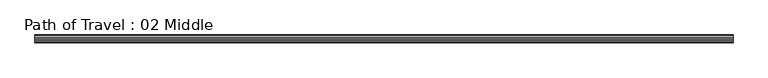
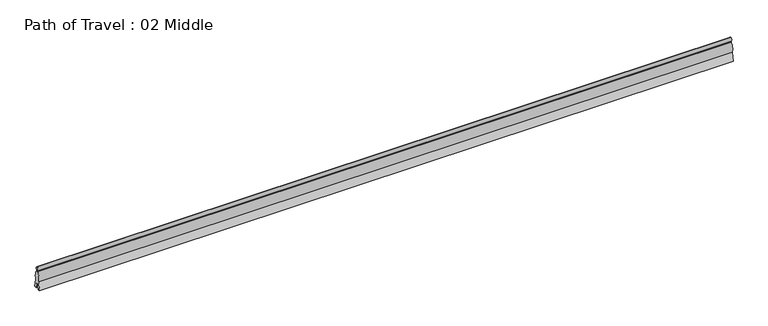
"""IFC4 building model written with IfcOpenShell, lengths in millimetres: proxy geometry, Path of Travel : 02 Middle."""

from ifc_helpers import new_model, si_unit, point, frame, origin, place, context, project, spatial, ellipse_curve, trimmed, source, transform, mapped, element, save
from ifc_brep_helpers import plane_surface, extruded_surface, advanced_brep


def path_of_travel_02_middle_d128f974(model_context):
    return source(origin(), model_context, "Body", "AdvancedBrep", [
        advanced_brep(
        [(227.5554837, 0.0, 1727.2), (227.5554837, 42.9018657, 1436.6534209), (227.5554837, 42.9018657, 1363.4763406), (227.5554837, 184.1186263, 643.4144547), (227.5554837, 297.5699544, 0.0), (227.5554837, 145.6574193, 0.0), (227.5554837, 0.0, 584.2), (227.5554837, -145.6574193, 0.0), (227.5554837, -297.5699544, 0.0), (227.5554837, -184.1186263, 643.4144547), (227.5554837, -42.9018657, 1363.4763406), (227.5554837, -42.9018657, 1436.6534209), (52272.1554837, 0.0, 1727.2), (52272.1554837, -42.9018657, 1436.6534209), (52272.1554837, -42.9018657, 1363.4763406), (52272.1554837, -184.1186263, 643.4144547), (52272.1554837, -297.5699544, 0.0), (52272.1554837, -145.6574193, 0.0), (52272.1554837, 0.0, 584.2), (52272.1554837, 145.6574193, 0.0), (52272.1554837, 297.5699544, 0.0), (52272.1554837, 184.1186263, 643.4144547), (52272.1554837, 42.9018657, 1363.4763406), (52272.1554837, 42.9018657, 1436.6534209)],
        [
            (0, 1, ellipse_curve(frame((227.5554837, 0.0, 1574.8), z_axis=(-1.0, 0.0, 0.0), x_axis=(0.0, 0.0, 1.0)), 152.4, 101.6)),
            (1, 2),
            (2, 3, ellipse_curve(frame((227.5554837, 0.0, 914.4), z_axis=(-1.0, 0.0, 0.0), x_axis=(0.0, 0.0, -1.0)), 457.2, 228.6)),
            (3, 4),
            (4, 5),
            (5, 6),
            (6, 7),
            (7, 8),
            (8, 9),
            (9, 10, ellipse_curve(frame((227.5554837, 0.0, 914.4), z_axis=(-1.0, 0.0, 0.0), x_axis=(0.0, 0.0, -1.0)), 457.2, 228.6)),
            (10, 11),
            (11, 0, ellipse_curve(frame((227.5554837, 0.0, 1574.8), z_axis=(-1.0, 0.0, 0.0), x_axis=(0.0, 0.0, 1.0)), 152.4, 101.6)),
            (12, 13, ellipse_curve(frame((52272.1554837, 0.0, 1574.8), z_axis=(1.0, 0.0, 0.0), x_axis=(0.0, 0.0, 1.0)), 152.4, 101.6)),
            (13, 14),
            (14, 15, ellipse_curve(frame((52272.1554837, 0.0, 914.4), z_axis=(1.0, 0.0, 0.0), x_axis=(0.0, 0.0, -1.0)), 457.2, 228.6)),
            (15, 16),
            (16, 17),
            (17, 18),
            (18, 19),
            (19, 20),
            (20, 21),
            (21, 22, ellipse_curve(frame((52272.1554837, 0.0, 914.4), z_axis=(1.0, 0.0, 0.0), x_axis=(0.0, 0.0, -1.0)), 457.2, 228.6)),
            (22, 23),
            (23, 12, ellipse_curve(frame((52272.1554837, 0.0, 1574.8), z_axis=(1.0, 0.0, 0.0), x_axis=(0.0, 0.0, 1.0)), 152.4, 101.6)),
            (0, 12),
            (23, 1),
            (22, 2),
            (21, 3),
            (20, 4),
            (19, 5),
            (18, 6),
            (17, 7),
            (16, 8),
            (15, 9),
            (14, 10),
            (13, 11),
        ],
        [
            plane_surface(frame((227.5554837, 0.0, 0.0), z_axis=(-1.0, 0.0, 0.0), x_axis=(0.0, 0.0, 1.0))),
            plane_surface(frame((52272.1554837, 0.0, 0.0), z_axis=(1.0, 0.0, 0.0), x_axis=(0.0, 0.0, 1.0))),
            extruded_surface(trimmed(ellipse_curve(frame((52272.1554837, 0.0, 1574.8), z_axis=(-1.0, 0.0, 0.0), x_axis=(0.0, 0.0, 1.0)), 152.4, 101.6), [point((52272.1554837, 0.0, 1727.2))], [point((52272.1554837, 42.9018657, 1436.6534209))], True, "CARTESIAN"), (-52044.6, 0.0, 0.0), 52044.6),
            plane_surface(frame((227.5554837, 42.9018657, 1436.6534209), z_axis=(0.0, 1.0, 0.0), x_axis=(1.0, 0.0, 0.0))),
            extruded_surface(trimmed(ellipse_curve(frame((52272.1554837, 0.0, 914.4), z_axis=(-1.0, 0.0, 0.0), x_axis=(0.0, 0.0, -1.0)), 457.2, 228.6), [point((52272.1554837, 42.9018657, 1363.4763406))], [point((52272.1554837, 184.1186263, 643.4144547))], True, "CARTESIAN"), (-52044.6, 0.0, 0.0), 52044.6),
            plane_surface(frame((227.5554837, 184.1186263, 643.4144547), z_axis=(0.0, 0.9848077530122078, 0.17364817766693205), x_axis=(1.0, 0.0, 0.0))),
            plane_surface(frame((227.5554837, 297.5699544, 0.0), z_axis=(0.0, 0.0, -1.0), x_axis=(1.0, 0.0, 0.0))),
            plane_surface(frame((227.5554837, 145.6574193, 0.0), z_axis=(0.0, -0.9702957262760199, -0.2419218955995739), x_axis=(1.0, 0.0, 0.0))),
            plane_surface(frame((227.5554837, 0.0, 584.2), z_axis=(0.0, 0.9702957262759961, -0.24192189559966923), x_axis=(1.0, 0.0, 0.0))),
            plane_surface(frame((227.5554837, -145.6574193, 0.0), z_axis=(0.0, 0.0, -1.0), x_axis=(1.0, 0.0, 0.0))),
            plane_surface(frame((227.5554837, -297.5699544, 0.0), z_axis=(0.0, -0.984807753012208, 0.17364817766693066), x_axis=(1.0, 0.0, 0.0))),
            extruded_surface(trimmed(ellipse_curve(frame((52272.1554837, 0.0, 914.4), z_axis=(-1.0, 0.0, 0.0), x_axis=(0.0, 0.0, -1.0)), 457.2, 228.6), [point((52272.1554837, -184.1186263, 643.4144547))], [point((52272.1554837, -42.9018657, 1363.4763406))], True, "CARTESIAN"), (-52044.6, 0.0, 0.0), 52044.6),
            plane_surface(frame((227.5554837, -42.9018657, 1363.4763406), z_axis=(0.0, -1.0, 0.0), x_axis=(1.0, 0.0, 0.0))),
            extruded_surface(trimmed(ellipse_curve(frame((52272.1554837, 0.0, 1574.8), z_axis=(-1.0, 0.0, 0.0), x_axis=(0.0, 0.0, 1.0)), 152.4, 101.6), [point((52272.1554837, -42.9018657, 1436.6534209))], [point((52272.1554837, 0.0, 1727.2))], True, "CARTESIAN"), (-52044.6, 0.0, 0.0), 52044.6),
        ],
        [
            (0, [[1, 2, 3, 4, 5, 6, 7, 8, 9, 10, 11, 12]]),
            (1, [[13, 14, 15, 16, 17, 18, 19, 20, 21, 22, 23, 24]]),
            (2, [[-1, 25, -24, 26]]),
            (3, [[-2, -26, -23, 27]]),
            (4, [[-3, -27, -22, 28]]),
            (5, [[-4, -28, -21, 29]]),
            (6, [[-5, -29, -20, 30]]),
            (7, [[-6, -30, -19, 31]]),
            (8, [[-7, -31, -18, 32]]),
            (9, [[-8, -32, -17, 33]]),
            (10, [[-9, -33, -16, 34]]),
            (11, [[-10, -34, -15, 35]]),
            (12, [[-11, -35, -14, 36]]),
            (13, [[-12, -36, -13, -25]]),
        ],
    ),
    ])


if __name__ == "__main__":
    model = new_model("IFC4")
    model_context = context("Model", 3, world=origin())
    ifc_project = project(units=[si_unit("LENGTHUNIT", "METRE", prefix="MILLI")], contexts=[model_context])
    site = spatial("IfcSite", under=ifc_project)
    building = spatial("IfcBuilding", under=site)
    placement = place(None, origin())
    path_of_travel_02_middle_shape = path_of_travel_02_middle_d128f974(model_context)
    element("IfcBuildingElementProxy", 1, Name="Path of Travel : 02 Middle", ObjectType="Path of Travel : 02 Middle", at=placement, inside=building, context=model_context, shape_type="MappedRepresentation", body=[
        mapped(path_of_travel_02_middle_shape, transform((0.0, 0.0, 0.0), x_axis=(1.0, 0.0, 0.0), y_axis=(0.0, 1.0, 0.0), z_axis=(0.0, 0.0, 1.0))),
    ])
    save(model, "model.ifc")

# Revit data of these elements
# Type "Path of Travel : 02 Middle"
#   Path of Egress [instance default] = 4' - 0"
#   built-in parameter 1001306 [instance default] = 4 (stored number, unit not read)
#   Dot at Start = no
#   Arrow in Middle = yes
#   Arrow at End = no
#   Egress Path = none
# Element 1 (IfcBuildingElementProxy, "Path of Travel : 02 Middle")
#   Path of Egress = 170' - 9"
#   built-in parameter 1001306 = 170.75 (stored number, unit not read)
#   Materials on its faces: "Egress Path Solid"
# Materials
#   "Egress Path Solid": class "Unassigned", colour RGB 255 128 64, transparency 0.75, Comments = "Rendering appearance not upgraded "
